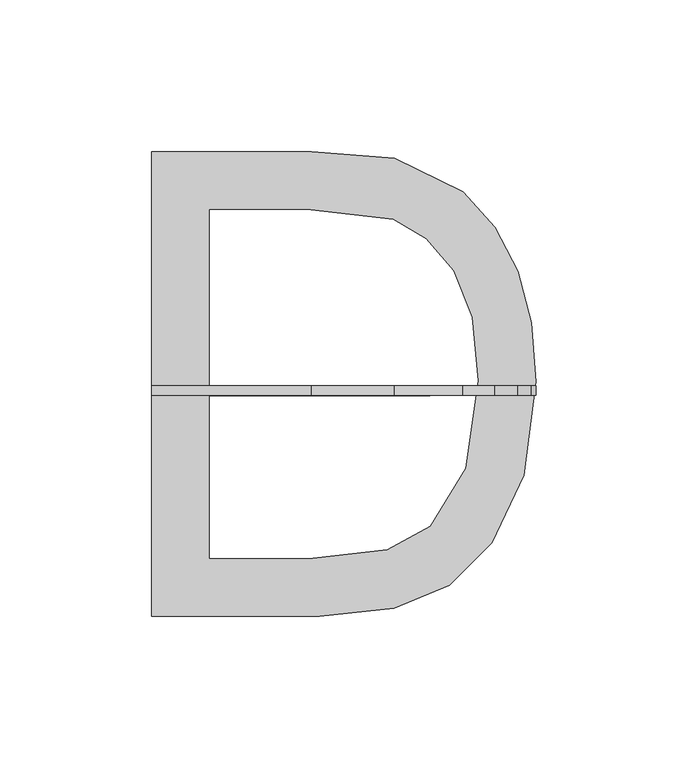
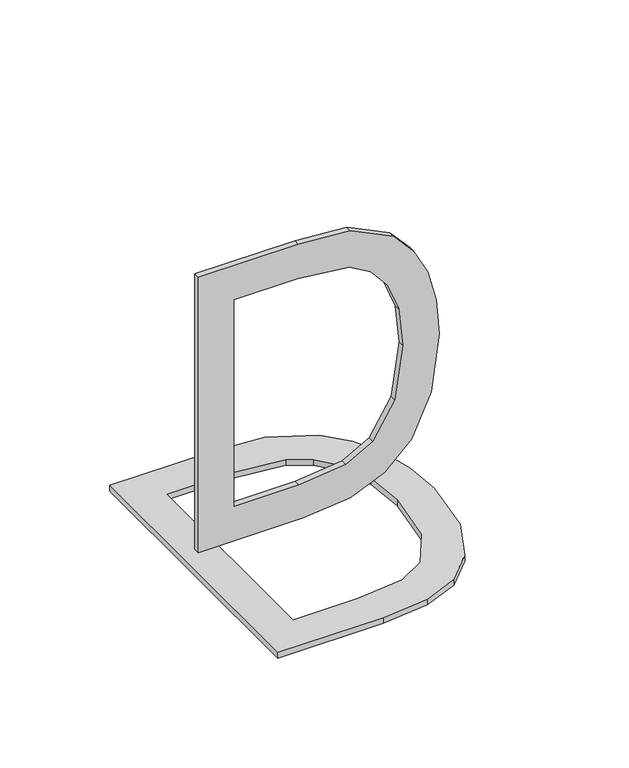
"""IFC4 building model written with IfcOpenShell, lengths in millimetres: proxy geometry, Grid Number1_FedEx : Grid Number1_FedEx."""

from ifc_helpers import new_model, si_unit, frame, origin, origin_with_axes, place, context, project, spatial, polyline, outline, extrude, source, transform, mapped, element, save


def entourage_a948333f(model_context):
    return source(origin(), model_context, "Body", "SweptSolid", [
        extrude(outline(polyline([(-167.8768239, 146.5840649), (-167.8768239, 299.6794816), (-115.0633903, 299.6794816), (-87.7409417, 297.4742498), (-65.2401017, 286.5228442), (-54.65312, 274.8612793), (-47.1123485, 260.3590767), (-42.5990986, 243.2965626), (-41.0946819, 223.9540631), (-45.1687543, 193.062129), (-55.6342613, 170.7668615), (-69.6131885, 156.8813763), (-87.9091374, 149.2004417), (-112.5217672, 146.5840649), (-167.8768239, 146.5840649)]), holes=[polyline([(-148.7398968, 165.720992), (-114.8765063, 165.720992), (-90.245188, 168.486876), (-76.042, 176.2986294), (-64.3991234, 195.3047377), (-60.231609, 224.2530776), (-62.2733173, 245.109338), (-68.3984422, 260.508584), (-77.4483025, 271.0862214), (-88.2642171, 277.477656), (-115.3997816, 280.5425545), (-148.7398968, 280.5425545), (-148.7398968, 165.720992)])]), origin_with_axes(), (0.0, 0.0, 1.0), 3.175),
        extrude(outline(polyline([(14.4798932, -167.8768239), (14.4798932, -112.5217672), (17.09627, -87.9091374), (24.7772046, -69.6131885), (38.6626898, -55.6342613), (60.9579574, -45.1687543), (91.8498914, -41.0946819), (111.192391, -42.5990986), (128.254905, -47.1123485), (142.7571076, -54.65312), (154.4186725, -65.2401017), (165.3700781, -87.7409417), (167.5753099, -115.0633903), (167.5753099, -167.8768239), (14.4798932, -167.8768239)]), holes=[polyline([(33.6168203, -148.7398968), (148.4383828, -148.7398968), (148.4383828, -115.3997816), (145.3734844, -88.2642171), (138.9820497, -77.4483025), (128.4044123, -68.3984422), (113.0051663, -62.2733173), (92.1489059, -60.231609), (63.200566, -64.3991234), (44.1944578, -76.042), (36.3827043, -90.245188), (33.6168203, -114.8765063), (33.6168203, -148.7398968)])]), frame((0.0, 219.3456765, 0.0), z_axis=(0.0, 1.0, 0.0), x_axis=(0.0, 0.0, 1.0)), (0.0, 0.0, 1.0), 3.175),
    ])


if __name__ == "__main__":
    model = new_model("IFC4")
    model_context = context("Model", 3, world=origin())
    ifc_project = project(units=[si_unit("LENGTHUNIT", "METRE", prefix="MILLI")], contexts=[model_context])
    site = spatial("IfcSite", under=ifc_project)
    building = spatial("IfcBuilding", under=site)
    placement = place(None, origin())
    entourage_shape = entourage_a948333f(model_context)
    element("IfcBuildingElementProxy", 1, Name="Grid Number1_FedEx : Grid Number1_FedEx", ObjectType="Grid Number1_FedEx : Grid Number1_FedEx", at=placement, inside=building, context=model_context, shape_type="MappedRepresentation", body=[
        mapped(entourage_shape, transform((0.0, 0.0, 0.0), x_axis=(1.0, 0.0, 0.0), y_axis=(0.0, 1.0, 0.0), z_axis=(0.0, 0.0, 1.0))),
    ])
    save(model, "model.ifc")

# Revit data of these elements
# Type "Grid Number1_FedEx : Grid Number1_FedEx"
#   Grid [instance default] = "S.8"
#   Label Width [instance default] = 1' - 0"
#   Half Box Width2 [instance default] = 0' - 6.13846"
#   Half Box Width [instance default] = 0' - 6"
#   Robust [instance default] = yes
#   Height = 0
#   Assembly Code = ""
# Element 1 (IfcBuildingElementProxy, "Grid Number1_FedEx : Grid Number1_FedEx")
#   Grid = "D"
#   Robust = no
#   Materials on its faces: "Letter"
# Materials
#   "Letter": class "Unassigned", colour RGB 178 187 30, transparency 0, Comments = "Rendering appearance not upgraded "
